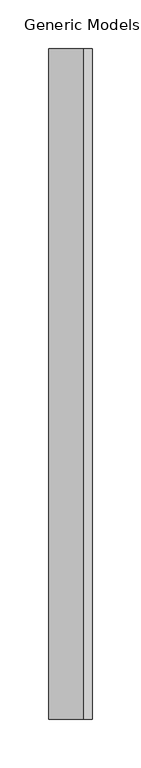
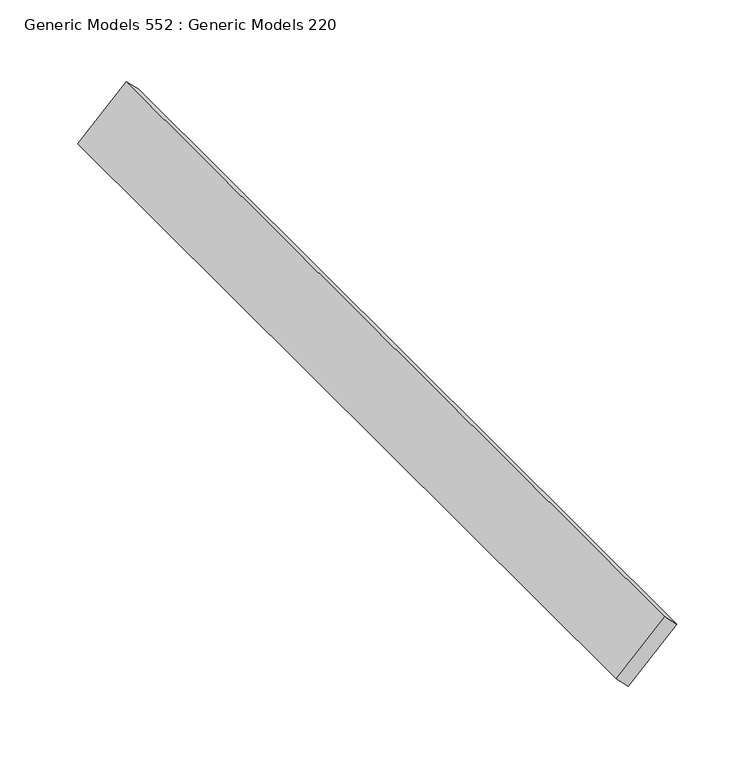
"""IFC4 building model written with IfcOpenShell, lengths in millimetres: proxy geometry, Generic Models 552 : Generic Models 220."""

from ifc_helpers import new_model, si_unit, frame, origin, place, context, project, spatial, polyline, outline, extrude, source, transform, mapped, element, save


def generic_models_552_generic_models_220_b659b1e2(model_context):
    return source(origin(), model_context, "Body", "SweptSolid", [
        extrude(outline(polyline([(0.0, -12.7000001), (0.0, 0.0), (690.8142348, 0.0), (690.8142348, -12.7000001), (0.0, -12.7000001)])), frame((7841.3059863, 4539.4872686, 124620.6399101), z_axis=(0.7071067811868034, 0.0, 0.7071067811862918), x_axis=(0.0, -1.0, 0.0)), (0.0, 0.0, 1.0), 50.8),
    ])


if __name__ == "__main__":
    model = new_model("IFC4")
    model_context = context("Model", 3, world=origin())
    ifc_project = project(units=[si_unit("LENGTHUNIT", "METRE", prefix="MILLI")], contexts=[model_context])
    site = spatial("IfcSite", under=ifc_project)
    building = spatial("IfcBuilding", under=site)
    placement = place(None, origin())
    generic_models_552_generic_models_220_shape = generic_models_552_generic_models_220_b659b1e2(model_context)
    element("IfcBuildingElementProxy", 1, Name="Generic Models 552 : Generic Models 220", ObjectType="Generic Models 552 : Generic Models 220", at=placement, inside=building, context=model_context, shape_type="MappedRepresentation", body=[
        mapped(generic_models_552_generic_models_220_shape, transform((0.0, 0.0, 0.0), x_axis=(1.0, 0.0, 0.0), y_axis=(0.0, 1.0, 0.0), z_axis=(0.0, 0.0, 1.0))),
    ])
    save(model, "model.ifc")

# Revit data of these elements
# Element 1 (IfcBuildingElementProxy, "Generic Models 552 : Generic Models 220")
#   Materials on its faces: "_WOOD TONE ALUMINUM EXTRUSION SLAT BY KNOTWOOD"
# Materials
#   "_WOOD TONE ALUMINUM EXTRUSION SLAT BY KNOTWOOD": class "Generic", colour RGB 177 130 114, transparency 0, Cost = 0
